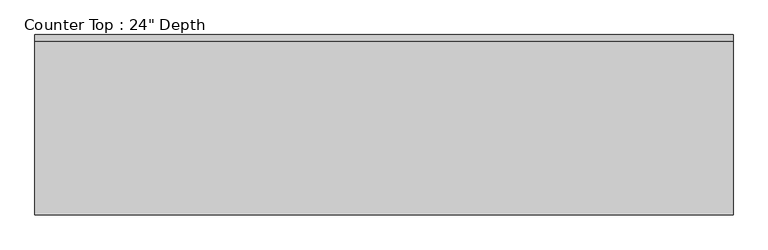
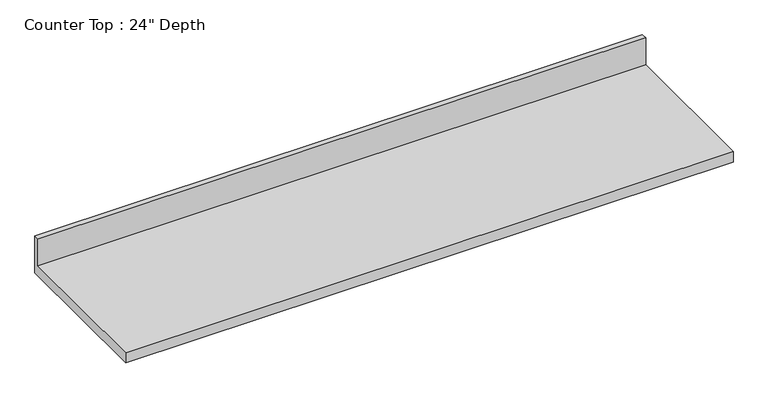
"""IFC4 building model written with IfcOpenShell, lengths in millimetres: furniture geometry."""

from ifc_helpers import new_model, si_unit, frame, origin, place, context, project, spatial, polyline, outline, extrude, source, transform, mapped, element, save


def furniture_2845e67d(model_context):
    return source(origin(), model_context, "Body", "SweptSolid", [
        extrude(outline(polyline([(0.0, 1016.0), (0.0, 876.3), (-558.8, 876.3), (-558.8, 914.4), (-19.05, 914.4), (-19.05, 1016.0), (0.0, 1016.0)])), frame((-1200.4622951, 0.0, 0.0), z_axis=(1.0, 0.0, 0.0), x_axis=(0.0, 1.0, 0.0)), (0.0, 0.0, 1.0), 2162.175),
    ])


if __name__ == "__main__":
    model = new_model("IFC4")
    model_context = context("Model", 3, world=origin())
    ifc_project = project(units=[si_unit("LENGTHUNIT", "METRE", prefix="MILLI")], contexts=[model_context])
    site = spatial("IfcSite", under=ifc_project)
    building = spatial("IfcBuilding", under=site)
    placement = place(None, origin())
    furniture_shape = furniture_2845e67d(model_context)
    element("IfcFurniture", 1, ObjectType="Counter Top : 24\" Depth", at=placement, inside=building, context=model_context, shape_type="MappedRepresentation", body=[
        mapped(furniture_shape, transform((0.0, 0.0, 0.0), x_axis=(1.0, 0.0, 0.0), y_axis=(0.0, 1.0, 0.0), z_axis=(0.0, 0.0, 1.0))),
    ])
    save(model, "model.ifc")

# Revit data of these elements
# Type "Counter Top : 24\" Depth"
#   Keynote = "M12366116.01"
#   Assembly Code = "C1030400"
#   Counter Thickness = 0' - 1 1/2"
#   Depth = 1' - 10"
#   Height = 3' - 0"
#   Length [instance default] = 8' - 0"
#   Counter Top Material = none
# Element 1 (IfcFurniture, "Counter Top : 24\" Depth")
#   Length = 7' - 1 1/8"
#   Materials on its faces: "CASEWORK"
# Materials
#   "CASEWORK": class "Generic", colour RGB 181 181 181, transparency 0, Cost = 0
